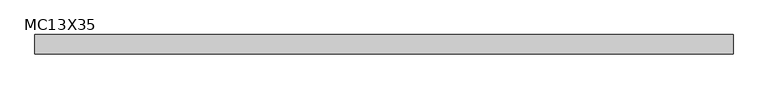
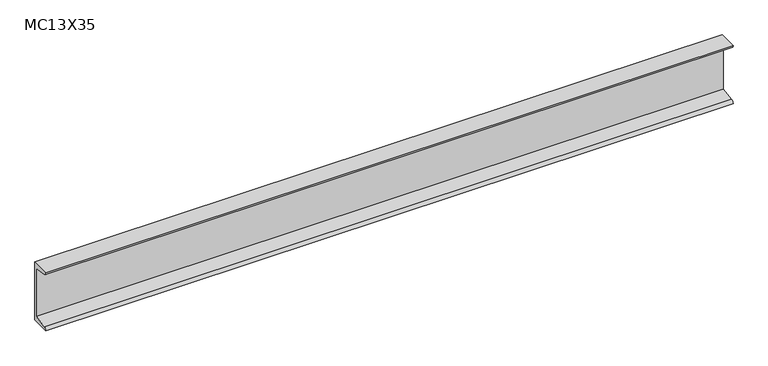
"""IFC4 building model written with IfcOpenShell, lengths in millimetres: beam geometry, MC-Miscellaneous Channel : MC13X35."""

from ifc_helpers import new_model, si_unit, point, frame, frame_2d, origin, place, context, project, spatial, polyline, circle_curve, trimmed, segment, composite_curve, outline, extrude, source, transform, mapped, element, save


def mc13x35_de2cde8a(model_context):
    return source(origin(), model_context, "Body", "SweptSolid", [
        extrude(outline(composite_curve([segment(polyline([(24.892, 165.1), (24.892, -165.1), (-78.486, -165.1)]), True, "CONTINUOUS"), segment(trimmed(circle_curve(frame_2d((-62.992, -165.1)), 15.494), [point((-78.486, -165.1))], [point((-62.992, -149.606))], False, "CARTESIAN"), True, "CONTINUOUS"), segment(polyline([(-62.992, -149.606), (13.5382, -137.4848071), (13.5382, 137.4848071), (-62.992, 149.606)]), True, "CONTINUOUS"), segment(trimmed(circle_curve(frame_2d((-62.992, 165.1)), 15.494), [point((-62.992, 149.606))], [point((-78.486, 165.1))], False, "CARTESIAN"), True, "CONTINUOUS"), segment(polyline([(-78.486, 165.1), (24.892, 165.1)]), True, "CONTINUOUS")], self_intersect=False)), frame((-1935.8893432, 0.0, 0.0), z_axis=(1.0, 0.0, 0.0), x_axis=(0.0, 1.0, 0.0)), (0.0, 0.0, 1.0), 3705.0911864),
    ])


if __name__ == "__main__":
    model = new_model("IFC4")
    model_context = context("Model", 3, world=origin())
    ifc_project = project(units=[si_unit("LENGTHUNIT", "METRE", prefix="MILLI")], contexts=[model_context])
    site = spatial("IfcSite", under=ifc_project)
    building = spatial("IfcBuilding", under=site)
    placement = place(None, origin())
    mc13x35_shape = mc13x35_de2cde8a(model_context)
    element("IfcBeam", 1, ObjectType="MC-Miscellaneous Channel : MC13X35", at=placement, inside=building, context=model_context, shape_type="MappedRepresentation", body=[
        mapped(mc13x35_shape, transform((0.0, 0.0, 0.0), x_axis=(1.0, 0.0, 0.0), y_axis=(0.0, 1.0, 0.0), z_axis=(0.0, 0.0, 1.0))),
    ])
    save(model, "model.ifc")

# Revit data of these elements
# Type "MC-Miscellaneous Channel : MC13X35"
#   Assembly Code = "B10"
#   W = 35
#   Length [instance default] = 5' - 0"
#   bf = 0' - 4.07"
#   d = 1' - 1"
#   tf = 0' - 0.61"
#   tw = 0' - 0.447"
#   x = 0' - 0.98"
#   A = 0.0715278 SF
#   Structural Material [instance default] = Steel ASTM A36
# Element 1 (IfcBeam, "MC-Miscellaneous Channel : MC13X35")
#   Structural Material = Steel ASTM A992
#   Materials on its faces: "Steel ASTM A992"
# Materials
#   "Steel ASTM A36": class "Metal", colour RGB 199 199 199, transparency 0, Description = "Structural steel, ASTM A36 Grade B, mill finish", Cost = 0
#   "Steel ASTM A992": class "Metal", colour RGB 199 199 199, transparency 0, Description = "Structural steel 50ksi", Cost = 0
